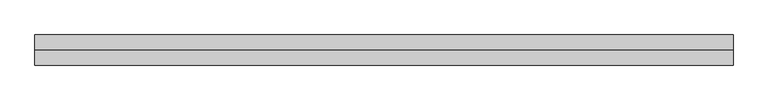
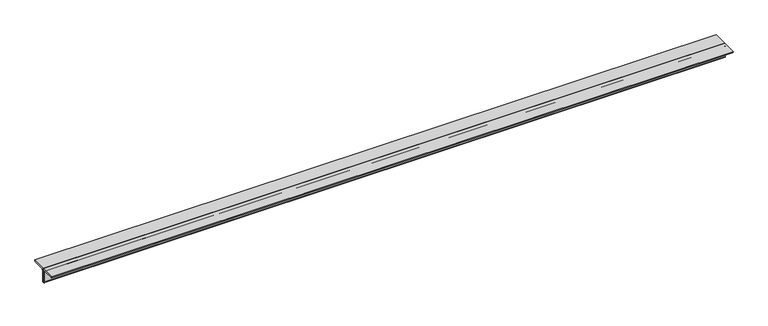
"""IFC4 building model written with IfcOpenShell, lengths in millimetres: member geometry, Steel Framing_2Ls_KS : H_SB_AR_S02_2Ls-100x100x10_VBR1."""

from ifc_helpers import new_model, si_unit, point, frame, frame_2d, origin, place, context, project, spatial, polyline, circle_curve, trimmed, segment, composite_curve, outline, extrude, source, transform, mapped, element, save


def member_0776a1bb(model_context):
    return source(origin(), model_context, "Body", "SweptSolid", [
        extrude(outline(composite_curve([segment(polyline([(0.0, 28.2), (100.0, 28.2)]), True, "CONTINUOUS"), segment(trimmed(circle_curve(frame_2d((90.0, 28.2)), 10.0), [point((100.0, 28.2))], [point((90.0, 18.2))], False, "CARTESIAN"), True, "CONTINUOUS"), segment(polyline([(90.0, 18.2), (20.0, 18.2)]), True, "CONTINUOUS"), segment(trimmed(circle_curve(frame_2d((20.0, 8.2)), 10.0), [point((20.0, 18.2))], [point((10.0, 8.2))], True, "CARTESIAN"), True, "CONTINUOUS"), segment(polyline([(10.0, 8.2), (10.0, -61.8)]), True, "CONTINUOUS"), segment(trimmed(circle_curve(frame_2d((0.0, -61.8)), 10.0), [point((10.0, -61.8))], [point((0.0, -71.8))], False, "CARTESIAN"), True, "CONTINUOUS"), segment(polyline([(0.0, -71.8), (0.0, 28.2)]), True, "CONTINUOUS")], self_intersect=False)), frame((-2190.4397751, 0.0, 0.0), z_axis=(1.0, 0.0, 0.0), x_axis=(0.0, 1.0, 0.0)), (0.0, 0.0, 1.0), 4633.0171831),
        extrude(outline(composite_curve([segment(polyline([(0.0, 28.2), (0.0, -71.8)]), True, "CONTINUOUS"), segment(trimmed(circle_curve(frame_2d((0.0, -61.8)), 10.0), [point((0.0, -71.8))], [point((-10.0, -61.8))], False, "CARTESIAN"), True, "CONTINUOUS"), segment(polyline([(-10.0, -61.8), (-10.0, 8.2)]), True, "CONTINUOUS"), segment(trimmed(circle_curve(frame_2d((-20.0, 8.2)), 10.0), [point((-10.0, 8.2))], [point((-20.0, 18.2))], True, "CARTESIAN"), True, "CONTINUOUS"), segment(polyline([(-20.0, 18.2), (-90.0, 18.2)]), True, "CONTINUOUS"), segment(trimmed(circle_curve(frame_2d((-90.0, 28.2)), 10.0), [point((-90.0, 18.2))], [point((-100.0, 28.2))], False, "CARTESIAN"), True, "CONTINUOUS"), segment(polyline([(-100.0, 28.2), (0.0, 28.2)]), True, "CONTINUOUS")], self_intersect=False)), frame((-2190.4397751, 0.0, 0.0), z_axis=(1.0, 0.0, 0.0), x_axis=(0.0, 1.0, 0.0)), (0.0, 0.0, 1.0), 4633.0171831),
    ])


if __name__ == "__main__":
    model = new_model("IFC4")
    model_context = context("Model", 3, world=origin())
    ifc_project = project(units=[si_unit("LENGTHUNIT", "METRE", prefix="MILLI")], contexts=[model_context])
    site = spatial("IfcSite", under=ifc_project)
    building = spatial("IfcBuilding", under=site)
    placement = place(None, origin())
    member_shape = member_0776a1bb(model_context)
    element("IfcMember", 1, ObjectType="Steel Framing_2Ls_KS : H_SB_AR_S02_2Ls-100x100x10_VBR1", at=placement, inside=building, context=model_context, shape_type="MappedRepresentation", body=[
        mapped(member_shape, transform((0.0, 0.0, 0.0), x_axis=(1.0, 0.0, 0.0), y_axis=(0.0, 1.0, 0.0), z_axis=(0.0, 0.0, 1.0))),
    ])
    save(model, "model.ifc")

# Revit data of these elements
# Type "Steel Framing_2Ls_KS : H_SB_AR_S02_2Ls-100x100x10_VBR1"
#   Type Comments = "MAIN"
#   Type Mark = "VBR1"
#   H_SectionID = "2Ls-100x100x10"
#   Assembly Code = "B10"
#   Legs = "LLBB"
#   H_Ratio for Additional Steel Plate = 0.2
#   W = 0
#   Perimeter = 0.80 m²/m
#   Nominal Weight = 29.80 kgf/m
#   Length [instance default] = 1524 mm
#   Space = 0 mm
#   b = 100 mm
#   d = 100 mm
#   t = 10 mm
#   y = 28.2 mm
#   A = 0.0038 m²
#   Structural Material [instance default] = Steel, 45-345
# Element 1 (IfcMember, "Steel Framing_2Ls_KS : H_SB_AR_S02_2Ls-100x100x10_VBR1")
#   Materials on its faces: "Steel, 45-345"
# Materials
#   "Steel, 45-345": class "Metal", colour RGB 189 187 185, transparency 0, Description = "Steel 345 MPa", Cost = 0
